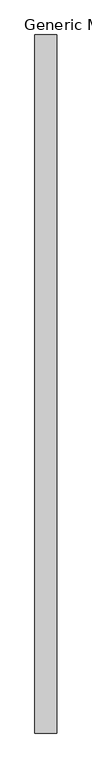
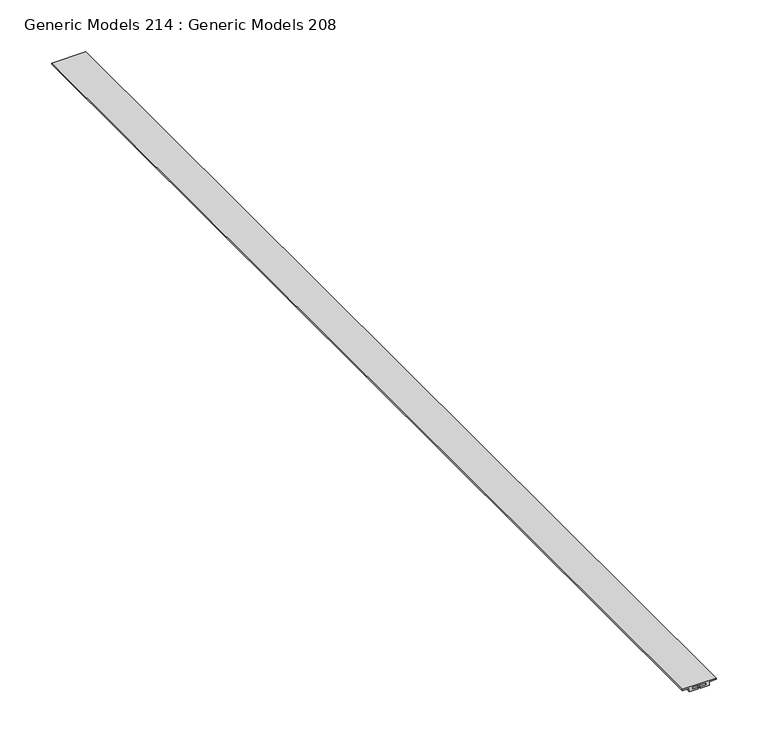
"""IFC4 building model written with IfcOpenShell, lengths in millimetres: proxy geometry, Generic Models 214 : Generic Models 208."""

from ifc_helpers import new_model, si_unit, frame, origin, place, context, project, spatial, polyline, outline, extrude, source, transform, mapped, element, save


def generic_models_214_generic_models_208_5dae2a39(model_context):
    return source(origin(), model_context, "Body", "SweptSolid", [
        extrude(outline(polyline([(2167.73125, 54439.7029264), (2167.73125, 54433.0042403), (2170.1125, 54433.0042403), (2170.1125, 54448.811695), (2167.73125, 54448.811695), (2167.73125, 54442.1130088), (2166.14375, 54442.1130088), (2166.14375, 54451.986695), (2170.1125, 54451.986695), (2170.1125, 54459.9579676), (2171.7, 54459.9579676), (2171.7, 54421.8579676), (2170.1125, 54421.8579676), (2170.1125, 54429.8292403), (2166.14375, 54429.8292403), (2166.14375, 54439.7029264), (2167.73125, 54439.7029264)])), frame((0.0, -228.7033818, 0.0), z_axis=(0.0, 1.0, 0.0), x_axis=(0.0, 0.0, 1.0)), (0.0, 0.0, 1.0), 1219.2),
    ])


if __name__ == "__main__":
    model = new_model("IFC4")
    model_context = context("Model", 3, world=origin())
    ifc_project = project(units=[si_unit("LENGTHUNIT", "METRE", prefix="MILLI")], contexts=[model_context])
    site = spatial("IfcSite", under=ifc_project)
    building = spatial("IfcBuilding", under=site)
    placement = place(None, origin())
    generic_models_214_generic_models_208_shape = generic_models_214_generic_models_208_5dae2a39(model_context)
    element("IfcBuildingElementProxy", 1, Name="Generic Models 214 : Generic Models 208", ObjectType="Generic Models 214 : Generic Models 208", at=placement, inside=building, context=model_context, shape_type="MappedRepresentation", body=[
        mapped(generic_models_214_generic_models_208_shape, transform((0.0, 0.0, 0.0), x_axis=(1.0, 0.0, 0.0), y_axis=(0.0, 1.0, 0.0), z_axis=(0.0, 0.0, 1.0))),
    ])
    save(model, "model.ifc")
